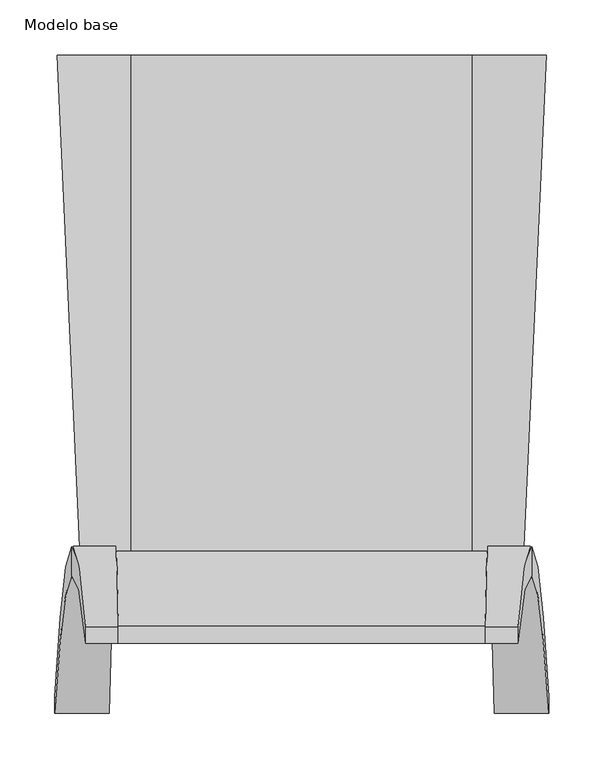
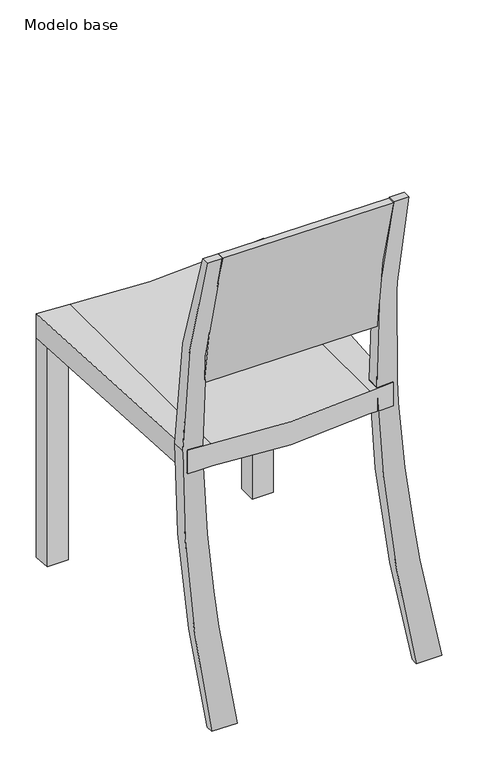
"""IFC4 building model written with IfcOpenShell, lengths in millimetres: furniture geometry, Silla - Madera (2) : Modelo base."""

from ifc_helpers import new_model, si_unit, frame, origin, origin_with_axes, place, context, project, spatial, polyline, circle_curve, ellipse_curve, outline, extrude, source, transform, mapped, element, save
from ifc_brep_helpers import plane_surface, cylinder_surface, revolved_surface, advanced_brep


def modelo_base_be08c04a(model_context):
    return source(origin(), model_context, "Body", "SolidModel", [
        advanced_brep(
        [(-167.062, -520.2637315, 922.805277), (-169.1260061, -451.6822204, 631.1538985), (-169.1260061, -476.85094, 631.1538985), (-167.062, -535.7344232, 922.805277), (167.0777417, -520.2637315, 920.4405823), (169.1428344, -451.6822204, 628.7599824), (169.1428344, -476.85094, 628.7599824), (167.0777417, -535.7344232, 920.4405823)],
        [
            (0, 1, circle_curve(frame((-169.8321061, -1530.470294, 531.3794559), z_axis=(-0.9999749592362468, 0.0, 0.007076786026638103), x_axis=(0.0025605874178329666, 0.9322444270823081, 0.36182008176171593)), 1083.3924247)),
            (1, 2),
            (2, 3, circle_curve(frame((-169.7736374, -1681.8941005, 539.6412969), z_axis=(0.9999749592362467, 0.0, -0.007076786026638103), x_axis=(-0.000231990271192452, 0.9994625301013882, -0.03278104793696645)), 1208.5131337)),
            (3, 0),
            (0, 4),
            (4, 5, ellipse_curve(frame((169.8493062, -1530.470294, 528.975543), z_axis=(-0.9999749378861258, 0.0, -0.007079802231631731), x_axis=(0.007079802231623589, 0.0, -0.9999749378861258)), 1083.5009963, 1083.3924247)),
            (5, 1),
            (5, 6),
            (6, 2),
            (6, 7, ellipse_curve(frame((169.7908067, -1681.8941005, 537.2382119), z_axis=(0.9999749378861258, 0.0, 0.007079802231631731), x_axis=(-0.007079802231623589, 0.0, 0.9999749378861257)), 1208.6342443, 1208.5131337)),
            (7, 3),
            (7, 4),
        ],
        [
            plane_surface(frame((-167.0579851, -520.4837438, 923.3725916), z_axis=(-0.9999749592362468, 0.0, 0.007076786026638008), x_axis=(0.0065972943349872325, -0.3618291422397858, 0.9322210829698492))),
            cylinder_surface(frame((-169.8321061, -1530.470294, 531.3794559), z_axis=(0.9999749592362468, 0.0, -0.007076786026638103), x_axis=(0.0025605874178329666, 0.9322444270823081, 0.36182008176171593)), 1083.3924247),
            plane_surface(frame((184.488376, -451.6822204, 628.6513825), z_axis=(-0.007076786026638094, 0.0, -0.9999749592362467), x_axis=(-0.9999749592362467, 0.0, 0.007076786026638094))),
            revolved_surface(polyline([(-170.05400070707284, -474.03050623144077, 500.02496993185025), (186.61972368744534, -474.03050623144077, 497.50080309592073)]), (-169.7736374, -1681.8941005, 539.6412969), (-0.9999749592362467, 0.0, 0.007076786026638103)),
            plane_surface(frame((186.552382, -535.7344232, 920.302761), z_axis=(0.007076786026638094, 0.0, 0.9999749592362467), x_axis=(-0.9999749592362467, 0.0, 0.007076786026638094))),
            plane_surface(frame((167.061, 43.0, 922.8052375), z_axis=(0.9999749378861258, 0.0, 0.007079802231631731), x_axis=(0.0, -1.0, 0.0))),
        ],
        [
            (0, [[1, 2, 3, 4]]),
            (1, [[5, 6, 7, -1]]),
            (2, [[-7, 8, 9, -2]]),
            (3, [[-9, 10, 11, -3]]),
            (4, [[-11, 12, -5, -4]]),
            (5, [[-12, -10, -8, -6]]),
        ],
    ),
        advanced_brep(
        [(224.9236272, -584.1809027, 3.307), (224.9236272, -598.919, 3.307), (175.2970931, -598.919, 3.307), (175.2970931, -584.1809027, 3.307), (209.6209787, -473.9604495, 502.2216956), (196.7208922, -535.7344266, 922.805275), (167.062, -535.7344266, 922.805275), (170.0540007, -474.0305027, 500.0249699), (170.0540007, -447.5154198, 500.0249699), (167.062, -520.483749, 922.805275), (196.7208922, -520.483749, 922.805275), (209.6209787, -447.4551966, 502.2216956)],
        [
            (0, 1),
            (1, 2),
            (2, 3),
            (3, 0),
            (1, 4, ellipse_curve(frame((208.4732537, -1681.8359776, 539.6411561), z_axis=(0.999529949707532, 0.0, 0.03065745647731721), x_axis=(-0.03065745647731806, 0.0, 0.999529949707532)), 1209.0233102, 1208.4550084)),
            (4, 5, ellipse_curve(frame((208.4732537, -1681.8359776, 539.6411561), z_axis=(0.999529949707532, 0.0, 0.03065745647731723), x_axis=(-0.03065745647731804, 0.0, 0.9995299497075321)), 1209.0233102, 1208.4550084)),
            (5, 6),
            (6, 7, ellipse_curve(frame((169.7736384, -1681.8359776, 539.6411561), z_axis=(-0.9999749592362469, 0.0, -0.007076786026603054), x_axis=(-0.007076786026602528, 0.0, 0.9999749592362469)), 1208.4852698, 1208.4550084)),
            (7, 2, ellipse_curve(frame((169.6358332, -1681.8359776, 539.6411561), z_axis=(-0.9999442956654316, 0.0, -0.010554883522048576), x_axis=(-0.010554883522032881, 0.0, 0.9999442956654316)), 1208.5223284, 1208.4550084)),
            (3, 8, ellipse_curve(frame((169.7290298, -1530.4189519, 530.8119297), z_axis=(0.9999442956654316, 0.0, 0.010554883522048576), x_axis=(0.010554883522032881, 0.0, -0.9999442956654316)), 1083.4014307, 1083.3410805)),
            (8, 9, ellipse_curve(frame((169.8361225, -1530.4189519, 530.8119297), z_axis=(0.9999749592362469, 0.0, 0.007076786026603054), x_axis=(0.007076786026602528, 0.0, -0.9999749592362469)), 1083.3682089, 1083.3410805)),
            (9, 10),
            (10, 11, ellipse_curve(frame((208.7440626, -1530.4189519, 530.8119297), z_axis=(-0.999529949707532, 0.0, -0.03065745647731723), x_axis=(0.03065745647731804, 0.0, -0.9995299497075321)), 1083.8505448, 1083.3410805)),
            (11, 0, ellipse_curve(frame((208.7440626, -1530.4189519, 530.8119297), z_axis=(-0.999529949707532, 0.0, -0.03065745647731721), x_axis=(0.03065745647731806, 0.0, -0.999529949707532)), 1083.8505448, 1083.3410805)),
            (7, 8),
            (6, 9),
            (5, 10),
            (4, 11),
        ],
        [
            plane_surface(frame((269.6998521, -584.1809027, 3.307), z_axis=(0.0, 0.0, -1.0), x_axis=(-1.0, 0.0, 0.0))),
            revolved_surface(polyline([(156.8800207899621, -2890.290986, 539.6411561), (245.53883321251948, -2890.290986, 539.6411561)]), (-284.9147268, -1681.8359776, 539.6411561), (-1.0, 0.0, 0.0)),
            cylinder_surface(frame((-284.9147268, -1530.4189519, 530.8119297), z_axis=(1.0, 0.0, 0.0), x_axis=(0.0, -1.0, 0.0)), 1083.3410805),
            plane_surface(frame((175.332, 43.0, 0.0), z_axis=(-0.9999442956654316, 0.0, -0.010554883522048576), x_axis=(0.0, -1.0, 0.0))),
            plane_surface(frame((170.0540007, 43.0, 500.0249699), z_axis=(-0.9999749592362469, 0.0, -0.007076786026603054), x_axis=(0.0, -1.0, 0.0))),
            plane_surface(frame((167.062, 43.0, 922.805275), z_axis=(0.0, 0.0, 1.0), x_axis=(0.0, -1.0, 0.0))),
            plane_surface(frame((196.7208922, 43.0, 922.805275), z_axis=(0.999529949707532, 0.0, 0.03065745647731723), x_axis=(0.0, -1.0, 0.0))),
            plane_surface(frame((209.6209787, 43.0, 502.2216956), z_axis=(0.999529949707532, 0.0, 0.03065745647731721), x_axis=(0.0, -1.0, 0.0))),
        ],
        [
            (0, [[1, 2, 3, 4]]),
            (1, [[5, 6, 7, 8, 9, -2]]),
            (2, [[10, 11, 12, 13, 14, -4]]),
            (3, [[-10, -3, -9, 15]]),
            (4, [[-8, 16, -11, -15]]),
            (5, [[-7, 17, -12, -16]]),
            (6, [[-6, 18, -13, -17]]),
            (7, [[-5, -1, -14, -18]]),
        ],
    ),
        advanced_brep(
        [(-175.2970931, -584.1809027, 3.307), (-175.2970931, -598.919, 3.307), (-224.9236272, -598.919, 3.307), (-224.9236272, -584.1809027, 3.307), (-170.0540007, -474.0305027, 500.0249699), (-167.062, -535.7344266, 922.805275), (-196.7208922, -535.7344266, 922.805275), (-209.6209787, -473.9604495, 502.2216956), (-209.6209787, -447.4551966, 502.2216956), (-196.7208922, -520.483749, 922.805275), (-167.062, -520.483749, 922.805275), (-170.0540007, -447.5154198, 500.0249699)],
        [
            (0, 1),
            (1, 2),
            (2, 3),
            (3, 0),
            (1, 4, ellipse_curve(frame((-169.6358332, -1681.8359776, 539.6411561), z_axis=(0.9999442956654323, 0.0, -0.010554883521987864), x_axis=(-0.010554883521967373, 0.0, -0.9999442956654325)), 1208.5223284, 1208.4550084)),
            (4, 5, ellipse_curve(frame((-169.7736384, -1681.8359776, 539.6411561), z_axis=(0.9999749592362467, 0.0, -0.007076786026638007), x_axis=(-0.007076786026630329, 0.0, -0.9999749592362467)), 1208.4852698, 1208.4550084)),
            (5, 6),
            (6, 7, ellipse_curve(frame((-208.4732537, -1681.8359776, 539.6411561), z_axis=(-0.999529949707532, 0.0, 0.030657456477317213), x_axis=(-0.030657456477318053, 0.0, -0.9995299497075318)), 1209.0233102, 1208.4550084)),
            (7, 2, ellipse_curve(frame((-208.4732537, -1681.8359776, 539.6411561), z_axis=(-0.999529949707532, 0.0, 0.03065745647731722), x_axis=(-0.030657456477318046, 0.0, -0.999529949707532)), 1209.0233102, 1208.4550084)),
            (3, 8, ellipse_curve(frame((-208.7440626, -1530.4189519, 530.8119297), z_axis=(0.999529949707532, 0.0, -0.03065745647731722), x_axis=(0.030657456477318046, 0.0, 0.999529949707532)), 1083.8505448, 1083.3410805)),
            (8, 9, ellipse_curve(frame((-208.7440626, -1530.4189519, 530.8119297), z_axis=(0.999529949707532, 0.0, -0.030657456477317213), x_axis=(0.030657456477318053, 0.0, 0.9995299497075318)), 1083.8505448, 1083.3410805)),
            (9, 10),
            (10, 11, ellipse_curve(frame((-169.8361225, -1530.4189519, 530.8119297), z_axis=(-0.9999749592362467, 0.0, 0.007076786026638007), x_axis=(0.007076786026630329, 0.0, 0.9999749592362467)), 1083.3682089, 1083.3410805)),
            (11, 0, ellipse_curve(frame((-169.7290298, -1530.4189519, 530.8119297), z_axis=(-0.9999442956654323, 0.0, 0.010554883521987864), x_axis=(0.010554883521967373, 0.0, 0.9999442956654325)), 1083.4014307, 1083.3410805)),
            (6, 9),
            (8, 7),
            (5, 10),
            (4, 11),
        ],
        [
            plane_surface(frame((269.6998521, -584.1809027, 3.307), z_axis=(0.0, 0.0, -1.0), x_axis=(-1.0, 0.0, 0.0))),
            revolved_surface(polyline([(-245.53883321251948, -2890.290986, 539.6411561), (-156.88002079004121, -2890.290986, 539.6411561)]), (-284.9147268, -1681.8359776, 539.6411561), (-1.0, 0.0, 0.0)),
            cylinder_surface(frame((-284.9147268, -1530.4189519, 530.8119297), z_axis=(1.0, 0.0, 0.0), x_axis=(0.0, -1.0, 0.0)), 1083.3410805),
            plane_surface(frame((-209.6209787, 43.0, 502.2216956), z_axis=(-0.999529949707532, 0.0, 0.030657456477317213), x_axis=(0.0, -1.0, 0.0))),
            plane_surface(frame((-196.7208922, 43.0, 922.805275), z_axis=(0.0, 0.0, 1.0), x_axis=(0.0, -1.0, 0.0))),
            plane_surface(frame((-167.062, 43.0, 922.805275), z_axis=(0.9999749592362467, 0.0, -0.007076786026638007), x_axis=(0.0, -1.0, 0.0))),
            plane_surface(frame((-170.0540007, 43.0, 500.0249699), z_axis=(0.9999442956654323, 0.0, -0.010554883521987864), x_axis=(0.0, -1.0, 0.0))),
            plane_surface(frame((-230.4680491, 43.0, -177.4586702), z_axis=(-0.999529949707532, 0.0, 0.03065745647731722), x_axis=(0.0, -1.0, 0.0))),
        ],
        [
            (0, [[1, 2, 3, 4]]),
            (1, [[5, 6, 7, 8, 9, -2]]),
            (2, [[10, 11, 12, 13, 14, -4]]),
            (3, [[-8, 15, -11, 16]]),
            (4, [[-7, 17, -12, -15]]),
            (5, [[-6, 18, -13, -17]]),
            (6, [[-5, -1, -14, -18]]),
            (7, [[-10, -3, -9, -16]]),
        ],
    ),
        advanced_brep(
        [(-222.6457845, 0.0, 453.04), (-222.6457845, 0.0, 502.944822), (-155.483, 0.0, 499.216), (155.483, 0.0, 499.216), (222.6457845, 0.0, 502.944822), (222.6457845, 0.0, 453.04), (179.6457845, 0.0, 453.04), (153.3625843, 0.0, 453.04), (-153.3625843, 0.0, 453.04), (-179.6457845, 0.0, 453.04), (-155.483, -476.488, 499.216), (-200.7915799, -476.488, 501.7314947), (-200.7915799, -476.488, 453.04), (-179.6457845, -476.488, 453.04), (-153.3625843, -476.488, 453.04), (153.3625843, -476.488, 453.04), (179.6457845, -476.488, 453.04), (200.7926448, -476.488, 453.04), (200.7926448, -476.488, 501.7315539), (155.483, -476.488, 499.216), (-202.123, -447.459, 453.04), (202.124, -447.459, 453.04), (202.124, -447.459, 501.8054696), (-202.123, -447.459, 501.8054141)],
        [
            (0, 1),
            (1, 2),
            (2, 3, circle_curve(frame((0.0, 0.0, 1957.3962887), z_axis=(0.0, -1.0, 0.0), x_axis=(1.0, 0.0, 0.0)), 1466.4462887)),
            (3, 4),
            (4, 5),
            (5, 6),
            (6, 7),
            (7, 8, circle_curve(frame((0.0, 0.0, 1620.8639519), z_axis=(0.0, 1.0, 0.0), x_axis=(1.0, 0.0, 0.0)), 1177.8509519)),
            (8, 9),
            (9, 0),
            (10, 11),
            (11, 12),
            (12, 13),
            (13, 14),
            (14, 15, circle_curve(frame((0.0, -476.488, 1620.8639519), z_axis=(0.0, -1.0, 0.0), x_axis=(1.0, 0.0, 0.0)), 1177.8509519)),
            (15, 16),
            (16, 17),
            (17, 18),
            (18, 19),
            (19, 10, circle_curve(frame((0.0, -476.488, 1957.3962887), z_axis=(0.0, 1.0, 0.0), x_axis=(1.0, 0.0, 0.0)), 1466.4462887)),
            (9, 13),
            (12, 20),
            (20, 0),
            (8, 14),
            (7, 15),
            (6, 16),
            (5, 21),
            (21, 17),
            (3, 19),
            (18, 22),
            (22, 4),
            (2, 10),
            (1, 23),
            (23, 11),
            (23, 20),
            (21, 22),
        ],
        [
            plane_surface(frame((-222.6457845, 0.0, 453.04), z_axis=(0.0, 1.0, 0.0), x_axis=(0.0, 0.0, -1.0))),
            plane_surface(frame((-222.6457845, -476.488, 453.04), z_axis=(0.0, -1.0, 0.0), x_axis=(0.0, 0.0, 1.0))),
            plane_surface(frame((-222.6457845, 0.0, 453.04), z_axis=(0.0, 0.0, -1.0), x_axis=(0.0, -1.0, 0.0))),
            plane_surface(frame((-179.6457845, 0.0, 453.04), z_axis=(0.0, 0.0, -1.0), x_axis=(0.0, -1.0, 0.0))),
            cylinder_surface(frame((0.0, -476.488, 1620.8639519), z_axis=(0.0, 1.0, 0.0), x_axis=(1.0, 0.0, 0.0)), 1177.8509519),
            plane_surface(frame((153.3625843, 0.0, 453.04), z_axis=(0.0, 0.0, -1.0), x_axis=(0.0, -1.0, 0.0))),
            plane_surface(frame((179.6457845, 0.0, 453.04), z_axis=(0.0, 0.0, -1.0), x_axis=(0.0, -1.0, 0.0))),
            plane_surface(frame((222.6457845, 0.0, 502.944822), z_axis=(-0.055433801494316516, 0.0, 0.9984623646647323), x_axis=(0.0, -1.0, 0.0))),
            revolved_surface(polyline([(1466.4462887, -476.488, 1957.3962887), (1466.4462887, 0.0, 1957.3962887)]), (0.0, -476.488, 1957.3962887), (0.0, -1.0, 0.0)),
            plane_surface(frame((-155.483, 0.0, 499.216), z_axis=(0.055433801494308495, 0.0, 0.9984623646647327), x_axis=(0.0, -1.0, 0.0))),
            plane_surface(frame((-202.123, -447.459, 708.9557379), z_axis=(-0.9989498494941665, -0.04581700771091594, 0.0), x_axis=(0.0, 0.0, -1.0))),
            plane_surface(frame((193.8773396, -627.2699913, 708.9557379), z_axis=(0.998949951670504, -0.04581477990231496, 0.0), x_axis=(0.0, 0.0, -1.0))),
            plane_surface(frame((202.124, -447.459, 708.9557379), z_axis=(0.998949951670504, -0.045814779902315125, 0.0), x_axis=(0.0, 0.0, -1.0))),
            plane_surface(frame((-222.6457845, 0.0, 708.9557379), z_axis=(-0.9989498494941665, -0.04581700771091578, 0.0), x_axis=(0.0, 0.0, -1.0))),
        ],
        [
            (0, [[1, 2, 3, 4, 5, 6, 7, 8, 9, 10]]),
            (1, [[11, 12, 13, 14, 15, 16, 17, 18, 19, 20]]),
            (2, [[21, -13, 22, 23, -10]]),
            (3, [[24, -14, -21, -9]]),
            (4, [[25, -15, -24, -8]]),
            (5, [[26, -16, -25, -7]]),
            (6, [[27, 28, -17, -26, -6]]),
            (7, [[29, -19, 30, 31, -4]]),
            (8, [[32, -20, -29, -3]]),
            (9, [[33, 34, -11, -32, -2]]),
            (10, [[-22, -12, -34, 35]]),
            (11, [[-30, -18, -28, 36]]),
            (12, [[-27, -5, -31, -36]]),
            (13, [[-33, -1, -23, -35]]),
        ],
    ),
        extrude(outline(polyline([(-179.6457845, -34.744), (-221.0522449, -34.744), (-222.6457845, 0.0), (-179.6457845, 0.0), (-179.6457845, -34.744)])), origin_with_axes(), (0.0, 0.0, 1.0), 453.04),
        extrude(outline(polyline([(179.6457845, 0.0), (222.6457845, 0.0), (221.0523225, -34.744), (179.6457845, -34.744), (179.6457845, 0.0)])), origin_with_axes(), (0.0, 0.0, 1.0), 453.04),
    ])


if __name__ == "__main__":
    model = new_model("IFC4")
    model_context = context("Model", 3, world=origin())
    ifc_project = project(units=[si_unit("LENGTHUNIT", "METRE", prefix="MILLI")], contexts=[model_context])
    site = spatial("IfcSite", under=ifc_project)
    building = spatial("IfcBuilding", under=site)
    placement = place(None, origin())
    modelo_base_shape = modelo_base_be08c04a(model_context)
    element("IfcFurniture", 1, ObjectType="Silla - Madera (2) : Modelo base", at=placement, inside=building, context=model_context, shape_type="MappedRepresentation", body=[
        mapped(modelo_base_shape, transform((0.0, 0.0, 0.0), x_axis=(1.0, 0.0, 0.0), y_axis=(0.0, 1.0, 0.0), z_axis=(0.0, 0.0, 1.0))),
    ])
    save(model, "model.ifc")

# Revit data of these elements
# Type "Silla - Madera (2) : Modelo base"
#   Máscara planta = yes
#   Máscara lateral = yes
#   Material = none
#   Manufacturer = ""
#   Default Elevation = 0
#   Assembly Code = ""
# Element 1 (IfcFurniture, "Silla - Madera (2) : Modelo base")
#   Materials on its faces: "Madera - Listel"
# Materials
#   "Madera - Listel": class "Madera", colour RGB 210 180 110, transparency 0, Cost = 0
